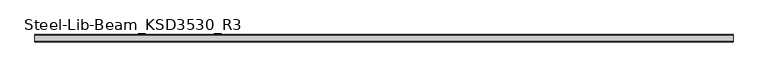
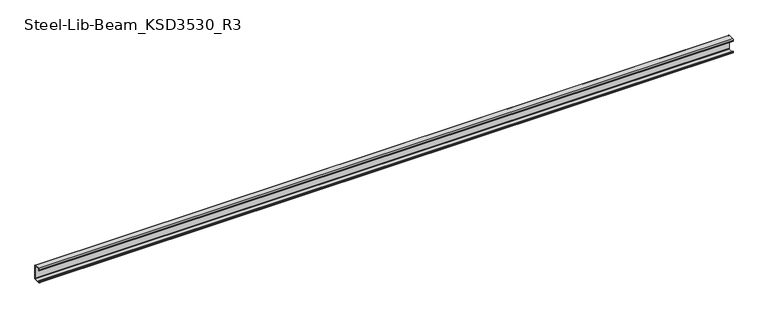
"""IFC4 building model written with IfcOpenShell, lengths in millimetres: beam geometry, Steel-Lib-Beam_KSD3530_R3 : BMS291_C-150×75x20x4.5."""

from ifc_helpers import new_model, si_unit, point, frame, frame_2d, origin, place, context, project, spatial, polyline, circle_curve, trimmed, segment, composite_curve, outline, extrude, source, transform, mapped, element, save


def steel_lib_beam_ksd3530_r3_8438cac7(model_context):
    return source(origin(), model_context, "Body", "SweptSolid", [
        extrude(outline(composite_curve([segment(trimmed(circle_curve(frame_2d((-41.0, 66.0)), 9.0), [point((-50.0, 66.0))], [point((-41.0, 75.0))], False, "CARTESIAN"), True, "CONTINUOUS"), segment(polyline([(-41.0, 75.0), (16.0, 75.0)]), True, "CONTINUOUS"), segment(trimmed(circle_curve(frame_2d((16.0, 66.0)), 9.0), [point((16.0, 75.0))], [point((25.0, 66.0))], False, "CARTESIAN"), True, "CONTINUOUS"), segment(polyline([(25.0, 66.0), (25.0, -66.0)]), True, "CONTINUOUS"), segment(trimmed(circle_curve(frame_2d((16.0, -66.0)), 9.0), [point((25.0, -66.0))], [point((16.0, -75.0))], False, "CARTESIAN"), True, "CONTINUOUS"), segment(polyline([(16.0, -75.0), (-41.0, -75.0)]), True, "CONTINUOUS"), segment(trimmed(circle_curve(frame_2d((-41.0, -66.0)), 9.0), [point((-41.0, -75.0))], [point((-50.0, -66.0))], False, "CARTESIAN"), True, "CONTINUOUS"), segment(polyline([(-50.0, -66.0), (-50.0, -55.0), (-45.5, -55.0), (-45.5, -66.0)]), True, "CONTINUOUS"), segment(trimmed(circle_curve(frame_2d((-41.0, -66.0)), 4.5), [point((-45.5, -66.0))], [point((-41.0, -70.5))], True, "CARTESIAN"), True, "CONTINUOUS"), segment(polyline([(-41.0, -70.5), (16.0, -70.5)]), True, "CONTINUOUS"), segment(trimmed(circle_curve(frame_2d((16.0, -66.0)), 4.5), [point((16.0, -70.5))], [point((20.5, -66.0))], True, "CARTESIAN"), True, "CONTINUOUS"), segment(polyline([(20.5, -66.0), (20.5, 66.0)]), True, "CONTINUOUS"), segment(trimmed(circle_curve(frame_2d((16.0, 66.0)), 4.5), [point((20.5, 66.0))], [point((16.0, 70.5))], True, "CARTESIAN"), True, "CONTINUOUS"), segment(polyline([(16.0, 70.5), (-41.0, 70.5)]), True, "CONTINUOUS"), segment(trimmed(circle_curve(frame_2d((-41.0, 66.0)), 4.5), [point((-41.0, 70.5))], [point((-45.5, 66.0))], True, "CARTESIAN"), True, "CONTINUOUS"), segment(polyline([(-45.5, 66.0), (-45.5, 55.0), (-50.0, 55.0), (-50.0, 66.0)]), True, "CONTINUOUS")], self_intersect=False)), frame((-3490.0, 0.0, 0.0), z_axis=(1.0, 0.0, 0.0), x_axis=(0.0, 1.0, 0.0)), (0.0, 0.0, 1.0), 6980.0),
    ])


if __name__ == "__main__":
    model = new_model("IFC4")
    model_context = context("Model", 3, world=origin())
    ifc_project = project(units=[si_unit("LENGTHUNIT", "METRE", prefix="MILLI")], contexts=[model_context])
    site = spatial("IfcSite", under=ifc_project)
    building = spatial("IfcBuilding", under=site)
    placement = place(None, origin())
    steel_lib_beam_ksd3530_r3_shape = steel_lib_beam_ksd3530_r3_8438cac7(model_context)
    element("IfcBeam", 1, ObjectType="Steel-Lib-Beam_KSD3530_R3 : BMS291_C-150×75x20x4.5", at=placement, inside=building, context=model_context, shape_type="MappedRepresentation", body=[
        mapped(steel_lib_beam_ksd3530_r3_shape, transform((0.0, 0.0, 0.0), x_axis=(1.0, 0.0, 0.0), y_axis=(0.0, 1.0, 0.0), z_axis=(0.0, 0.0, 1.0))),
    ])
    save(model, "model.ifc")

# Revit data of these elements
# Type "Steel-Lib-Beam_KSD3530_R3 : BMS291_C-150×75x20x4.5"
#   Keynote = "C-150×75x20x4.5"
#   SteelWeight = "Light"
#   x = 0.0250 m
#   t1 = 0.0090 m
#   t = 0.0045 m
#   Surface Area = 0.629834 m²/m
#   Section Area = 13.9688 cm²
#   Mass per Unit Length = 10.9655 kg/m
#   C = 0.0200 m
#   A = 0.0750 m
#   Length [instance default] = 1.5000 m
#   H = 0.1500 m
#   hec_material4 [instance default] = none
#   hec_material3 [instance default] = none
#   hec_material2 [instance default] = none
#   hec_material1 [instance default] = none
#   Structural Material [instance default] = Metal - Steel - Light Gauge
#   Assembly Code = ""
# Element 1 (IfcBeam, "Steel-Lib-Beam_KSD3530_R3 : BMS291_C-150×75x20x4.5")
#   Structural Material = none
# Materials
#   "Metal - Steel - Light Gauge": class "Metal", colour RGB 247 247 247, transparency 0
